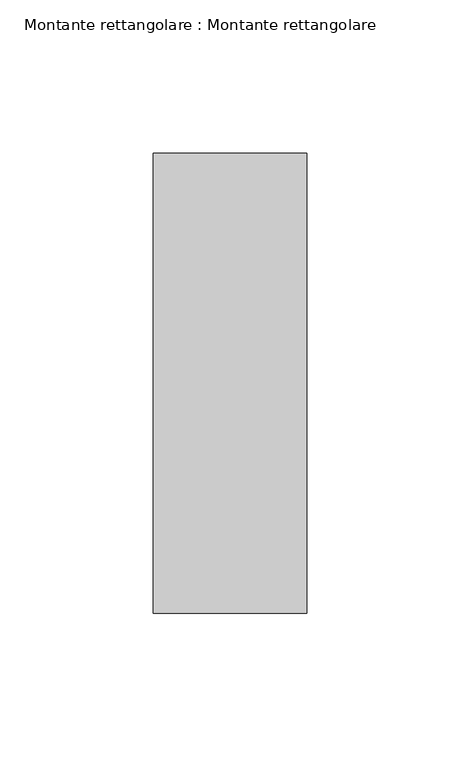
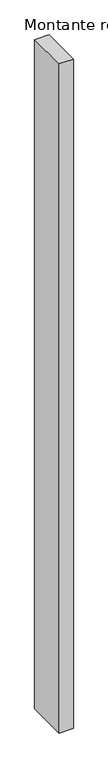
"""IFC4 building model written with IfcOpenShell, lengths in millimetres: member geometry, Montante rettangolare : Montante rettangolare."""

from ifc_helpers import new_model, si_unit, frame, origin, place, context, project, spatial, polyline, outline, extrude, source, transform, mapped, element, save


def montante_rettangolare_montante_rettangolare_eb9201c3(model_context):
    return source(origin(), model_context, "Body", "SweptSolid", [
        extrude(outline(polyline([(25.0, 75.0), (25.0, -75.0), (-25.0, -75.0), (-25.0, 75.0), (25.0, 75.0)])), frame((0.0, 0.0, -2500.0), z_axis=(0.0, 0.0, 1.0), x_axis=(1.0, 0.0, 0.0)), (0.0, 0.0, 1.0), 2500.0),
    ])


if __name__ == "__main__":
    model = new_model("IFC4")
    model_context = context("Model", 3, world=origin())
    ifc_project = project(units=[si_unit("LENGTHUNIT", "METRE", prefix="MILLI")], contexts=[model_context])
    site = spatial("IfcSite", under=ifc_project)
    building = spatial("IfcBuilding", under=site)
    placement = place(None, origin())
    montante_rettangolare_montante_rettangolare_shape = montante_rettangolare_montante_rettangolare_eb9201c3(model_context)
    element("IfcMember", 1, ObjectType="Montante rettangolare : Montante rettangolare", at=placement, inside=building, context=model_context, shape_type="MappedRepresentation", body=[
        mapped(montante_rettangolare_montante_rettangolare_shape, transform((0.0, 0.0, 0.0), x_axis=(1.0, 0.0, 0.0), y_axis=(0.0, 1.0, 0.0), z_axis=(0.0, 0.0, 1.0))),
    ])
    save(model, "model.ifc")

# Revit data of these elements
# Type "Montante rettangolare : Montante rettangolare"
#   built-in parameter 1007304 = 0.492126 (stored number, unit not read)
#   built-in parameter 1007301 = 0.082021 (stored number, unit not read)
#   built-in parameter 1007300 = 0.082021 (stored number, unit not read)
# Element 1 (IfcMember, "Montante rettangolare : Montante rettangolare")
#   Materials on its faces: "Acciaio"
# Materials
#   "Acciaio": class "Metallo", colour RGB 247 247 247, transparency 0, Description = "Acciaio, finitura zigrinata", Cost = 0
